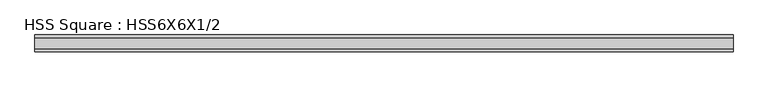
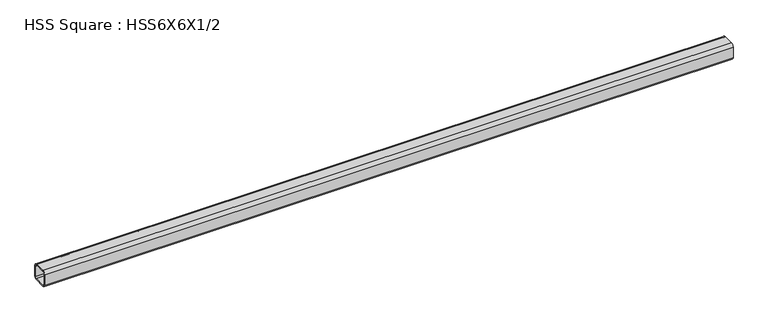
"""IFC4 building model written with IfcOpenShell, lengths in millimetres: member geometry, HSS Square : HSS6X6X1/2."""

from ifc_helpers import new_model, si_unit, point, frame, frame_2d, origin, place, context, project, spatial, polyline, circle_curve, trimmed, segment, composite_curve, outline, extrude, source, transform, mapped, element, save


def hss_square_hss6x6x1_2_5971bc98(model_context):
    return source(origin(), model_context, "Body", "SweptSolid", [
        extrude(outline(composite_curve([segment(polyline([(76.2, 50.8), (76.2, -50.8)]), True, "CONTINUOUS"), segment(trimmed(circle_curve(frame_2d((50.8, -50.8)), 25.4), [point((76.2, -50.8))], [point((50.8, -76.2))], False, "CARTESIAN"), True, "CONTINUOUS"), segment(polyline([(50.8, -76.2), (-50.8, -76.2)]), True, "CONTINUOUS"), segment(trimmed(circle_curve(frame_2d((-50.8, -50.8)), 25.4), [point((-50.8, -76.2))], [point((-76.2, -50.8))], False, "CARTESIAN"), True, "CONTINUOUS"), segment(polyline([(-76.2, -50.8), (-76.2, 50.8)]), True, "CONTINUOUS"), segment(trimmed(circle_curve(frame_2d((-50.8, 50.8)), 25.4), [point((-76.2, 50.8))], [point((-50.8, 76.2))], False, "CARTESIAN"), True, "CONTINUOUS"), segment(polyline([(-50.8, 76.2), (50.8, 76.2)]), True, "CONTINUOUS"), segment(trimmed(circle_curve(frame_2d((50.8, 50.8)), 25.4), [point((50.8, 76.2))], [point((76.2, 50.8))], False, "CARTESIAN"), True, "CONTINUOUS")], self_intersect=False), holes=[composite_curve([segment(trimmed(circle_curve(frame_2d((-50.8, 50.8)), 12.7), [point((-50.8, 63.5))], [point((-63.5, 50.8))], True, "CARTESIAN"), True, "CONTINUOUS"), segment(polyline([(-63.5, 50.8), (-63.5, -50.8)]), True, "CONTINUOUS"), segment(trimmed(circle_curve(frame_2d((-50.8, -50.8)), 12.7), [point((-63.5, -50.8))], [point((-50.8, -63.5))], True, "CARTESIAN"), True, "CONTINUOUS"), segment(polyline([(-50.8, -63.5), (50.8, -63.5)]), True, "CONTINUOUS"), segment(trimmed(circle_curve(frame_2d((50.8, -50.8)), 12.7), [point((50.8, -63.5))], [point((63.5, -50.8))], True, "CARTESIAN"), True, "CONTINUOUS"), segment(polyline([(63.5, -50.8), (63.5, 50.8)]), True, "CONTINUOUS"), segment(trimmed(circle_curve(frame_2d((50.8, 50.8)), 12.7), [point((63.5, 50.8))], [point((50.8, 63.5))], True, "CARTESIAN"), True, "CONTINUOUS"), segment(polyline([(50.8, 63.5), (-50.8, 63.5)]), True, "CONTINUOUS")], self_intersect=False)]), frame((-3151.9009315, 0.0, 0.0), z_axis=(1.0, 0.0, 0.0), x_axis=(0.0, 1.0, 0.0)), (0.0, 0.0, 1.0), 6303.8018631),
    ])


if __name__ == "__main__":
    model = new_model("IFC4")
    model_context = context("Model", 3, world=origin())
    ifc_project = project(units=[si_unit("LENGTHUNIT", "METRE", prefix="MILLI")], contexts=[model_context])
    site = spatial("IfcSite", under=ifc_project)
    building = spatial("IfcBuilding", under=site)
    placement = place(None, origin())
    hss_square_hss6x6x1_2_shape = hss_square_hss6x6x1_2_5971bc98(model_context)
    element("IfcMember", 1, ObjectType="HSS Square : HSS6X6X1/2", at=placement, inside=building, context=model_context, shape_type="MappedRepresentation", body=[
        mapped(hss_square_hss6x6x1_2_shape, transform((0.0, 0.0, 0.0), x_axis=(1.0, 0.0, 0.0), y_axis=(0.0, 1.0, 0.0), z_axis=(0.0, 0.0, 1.0))),
    ])
    save(model, "model.ifc")

# Revit data of these elements
# Type "HSS Square : HSS6X6X1/2"
#   Section Name Key = "HSS 6X6X1/2"
#   Assembly Code = "B10"
#   Width = 6.000"
#   Wall Nominal Thickness = 0.500"
#   Wall Design Thickness = 0.465"
#   Torsional Moment of Inertia = 81.10 in⁴
#   Torsional Modulus = 28.10 in³
#   Section Area = 9.74 in²
#   Plastic Modulus weak axis = 19.80 in³
#   Plastic Modulus strong axis = 19.80 in³
#   Outer Fillet = 1.000"
#   Nominal Weight = 35.24 lbf/ft
#   Moment of Inertia weak axis = 48.30 in⁴
#   Moment of Inertia strong axis = 48.30 in⁴
#   Inner Fillet = 0.500"
#   Height = 6.000"
#   Elastic Modulus weak axis = 16.10 in³
#   Elastic Modulus strong axis = 16.10 in³
#   Centroid Vertical = 3.000"
#   Centroid Horizontal = 3.000"
#   Length [instance default] = 5' - 0"
#   Structural Material [instance default] = Steel ASTM A500, Grade B, Rectangular and Square
#   Principal Axes Angle = 0
# Element 1 (IfcMember, "HSS Square : HSS6X6X1/2")
#   Structural Material = Steel ASTM A36
#   Materials on its faces: "Steel ASTM A36"
# Materials
#   "Steel ASTM A500, Grade B, Rectangular and Square": class "Metal", colour RGB 199 199 199, transparency 0, Description = "Carbon steel", Cost = 0
#   "Steel ASTM A36": class "Metal", colour RGB 199 199 199, transparency 0, Description = "Structural steel, ASTM A36 Grade B, mill finish", Cost = 0
